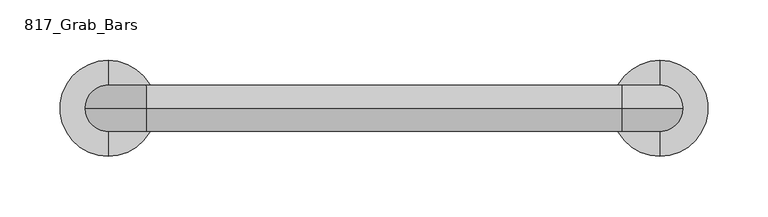
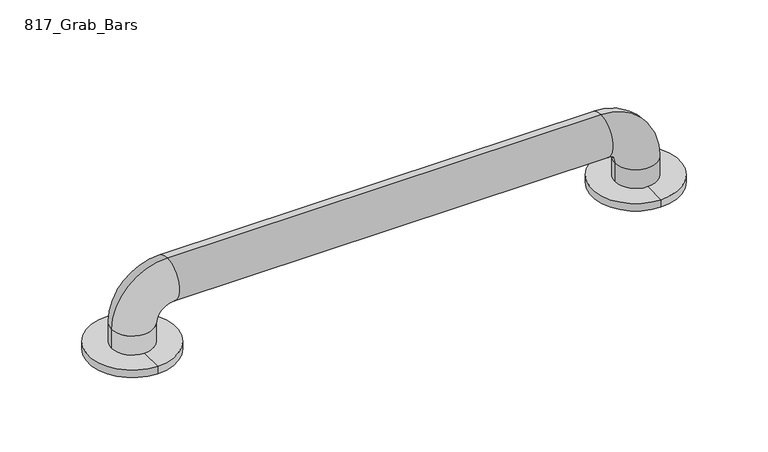
"""IFC4 building model written with IfcOpenShell, lengths in millimetres: proxy geometry, 817_Grab_Bars : 8170-001180."""

from ifc_helpers import new_model, si_unit, point, frame, origin, place, context, project, spatial, circle_curve, ellipse_curve, trimmed, source, transform, mapped, element, save
from ifc_brep_helpers import plane_surface, cylinder_surface, revolved_surface, advanced_brep


def proxy_817_grab_bars_5335159d(model_context):
    return source(origin(), model_context, "Body", "AdvancedBrep", [
        advanced_brep(
        [(-134.9375, -496.8875, 7.14375), (-134.9375, -576.2625, 7.14375), (-134.9375, -555.625, 7.14375), (-153.9875, -536.575, 7.14375), (-134.9375, -517.525, 7.14375), (-115.8875, -536.575, 7.14375), (-134.9375, -576.2625, 0.0), (-134.9375, -496.8875, 0.0), (-134.9375, -517.525, 0.0), (-134.9375, -536.575, 0.0), (-134.9375, -555.625, 0.0), (322.2625, -496.8875, 7.14375), (322.2625, -576.2625, 7.14375), (322.2625, -555.625, 7.14375), (303.2125, -536.575, 7.14375), (322.2625, -517.525, 7.14375), (341.3125, -536.575, 7.14375), (322.2625, -576.2625, 0.0), (322.2625, -496.8875, 0.0), (322.2625, -517.525, 0.0), (322.2625, -536.575, 0.0), (322.2625, -555.625, 0.0), (-153.9875, -536.575, 25.4), (-115.8875, -536.575, 25.4), (-103.1875, -536.575, 76.2), (-103.1875, -536.575, 38.1), (290.5125, -536.575, 76.2), (290.5125, -536.575, 38.1), (341.3125, -536.575, 25.4), (303.2125, -536.575, 25.4)],
        [
            (0, 1, circle_curve(frame((-134.9375, -536.575, 7.14375), z_axis=(0.0, 0.0, 1.0), x_axis=(0.0, 1.0, 0.0)), 39.6875)),
            (1, 2),
            (2, 3, circle_curve(frame((-134.9375, -536.575, 7.14375), z_axis=(0.0, 0.0, -1.0), x_axis=(1.0, 0.0, 0.0)), 19.05)),
            (3, 4, circle_curve(frame((-134.9375, -536.575, 7.14375), z_axis=(0.0, 0.0, -1.0), x_axis=(1.0, 0.0, 0.0)), 19.05)),
            (4, 0),
            (1, 0, circle_curve(frame((-134.9375, -536.575, 7.14375), z_axis=(0.0, 0.0, 1.0), x_axis=(0.0, 1.0, 0.0)), 39.6875)),
            (4, 5, circle_curve(frame((-134.9375, -536.575, 7.14375), z_axis=(0.0, 0.0, -1.0), x_axis=(1.0, 0.0, 0.0)), 19.05)),
            (5, 2, circle_curve(frame((-134.9375, -536.575, 7.14375), z_axis=(0.0, 0.0, -1.0), x_axis=(1.0, 0.0, 0.0)), 19.05)),
            (6, 7, circle_curve(frame((-134.9375, -536.575, 0.0), z_axis=(0.0, 0.0, -1.0), x_axis=(0.0, 1.0, 0.0)), 39.6875)),
            (7, 8),
            (8, 9),
            (9, 10),
            (10, 6),
            (7, 6, circle_curve(frame((-134.9375, -536.575, 0.0), z_axis=(0.0, 0.0, -1.0), x_axis=(0.0, 1.0, 0.0)), 39.6875)),
            (0, 7),
            (6, 1),
            (11, 12, circle_curve(frame((322.2625, -536.575, 7.14375), z_axis=(0.0, 0.0, 1.0), x_axis=(0.0, 1.0, 0.0)), 39.6875)),
            (12, 13),
            (13, 14, circle_curve(frame((322.2625, -536.575, 7.14375), z_axis=(0.0, 0.0, -1.0), x_axis=(-1.0, 0.0, 0.0)), 19.05)),
            (14, 15, circle_curve(frame((322.2625, -536.575, 7.14375), z_axis=(0.0, 0.0, -1.0), x_axis=(-1.0, 0.0, 0.0)), 19.05)),
            (15, 11),
            (12, 11, circle_curve(frame((322.2625, -536.575, 7.14375), z_axis=(0.0, 0.0, 1.0), x_axis=(0.0, 1.0, 0.0)), 39.6875)),
            (15, 16, circle_curve(frame((322.2625, -536.575, 7.14375), z_axis=(0.0, 0.0, -1.0), x_axis=(-1.0, 0.0, 0.0)), 19.05)),
            (16, 13, circle_curve(frame((322.2625, -536.575, 7.14375), z_axis=(0.0, 0.0, -1.0), x_axis=(-1.0, 0.0, 0.0)), 19.05)),
            (17, 18, circle_curve(frame((322.2625, -536.575, 0.0), z_axis=(0.0, 0.0, -1.0), x_axis=(0.0, 1.0, 0.0)), 39.6875)),
            (18, 19),
            (19, 20),
            (20, 21),
            (21, 17),
            (18, 17, circle_curve(frame((322.2625, -536.575, 0.0), z_axis=(0.0, 0.0, -1.0), x_axis=(0.0, 1.0, 0.0)), 39.6875)),
            (11, 18),
            (17, 12),
            (22, 23, circle_curve(frame((-134.9375, -536.575, 25.4), z_axis=(0.0, 0.0, -1.0), x_axis=(1.0, 0.0, 0.0)), 19.05)),
            (23, 5),
            (3, 22),
            (23, 22, circle_curve(frame((-134.9375, -536.575, 25.4), z_axis=(0.0, 0.0, -1.0), x_axis=(1.0, 0.0, 0.0)), 19.05)),
            (22, 24, circle_curve(frame((-103.1875, -536.575, 25.4), z_axis=(0.0, 1.0, 0.0), x_axis=(-1.0, 0.0, 0.0)), 50.8)),
            (24, 25, circle_curve(frame((-103.1875, -536.575, 57.15), z_axis=(-1.0, 0.0, 0.0), x_axis=(0.0, 0.0, -1.0)), 19.05)),
            (25, 23, circle_curve(frame((-103.1875, -536.575, 25.4), z_axis=(0.0, -1.0, 0.0), x_axis=(-1.0, 0.0, 0.0)), 12.7)),
            (25, 24, circle_curve(frame((-103.1875, -536.575, 57.15), z_axis=(-1.0, 0.0, 0.0), x_axis=(0.0, 0.0, -1.0)), 19.05)),
            (24, 26),
            (26, 27, circle_curve(frame((290.5125, -536.575, 57.15), z_axis=(-1.0, 0.0, 0.0), x_axis=(0.0, 0.0, -1.0)), 19.05)),
            (27, 25),
            (27, 26, circle_curve(frame((290.5125, -536.575, 57.15), z_axis=(-1.0, 0.0, 0.0), x_axis=(0.0, 0.0, -1.0)), 19.05)),
            (26, 28, circle_curve(frame((290.5125, -536.575, 25.4), z_axis=(0.0, 1.0, 0.0), x_axis=(0.0, 0.0, 1.0)), 50.8)),
            (28, 29, circle_curve(frame((322.2625, -536.575, 25.4), z_axis=(0.0, 0.0, 1.0), x_axis=(-1.0, 0.0, 0.0)), 19.05)),
            (29, 27, circle_curve(frame((290.5125, -536.575, 25.4), z_axis=(0.0, -1.0, 0.0), x_axis=(0.0, 0.0, 1.0)), 12.7)),
            (29, 28, circle_curve(frame((322.2625, -536.575, 25.4), z_axis=(0.0, 0.0, 1.0), x_axis=(-1.0, 0.0, 0.0)), 19.05)),
            (28, 16),
            (14, 29),
        ],
        [
            plane_surface(frame((-134.9375, -536.575, 7.14375), z_axis=(0.0, 0.0, 1.0), x_axis=(0.0, 1.0, 0.0))),
            plane_surface(frame((-134.9375, -536.575, 0.0), z_axis=(0.0, 0.0, -1.0), x_axis=(0.0, 1.0, 0.0))),
            cylinder_surface(frame((-134.9375, -536.575, 7.14375), z_axis=(0.0, 0.0, 1.0), x_axis=(0.0, 1.0, 0.0)), 39.6875),
            plane_surface(frame((322.2625, -536.575, 7.14375), z_axis=(0.0, 0.0, 1.0), x_axis=(0.0, 1.0, 0.0))),
            plane_surface(frame((322.2625, -536.575, 0.0), z_axis=(0.0, 0.0, -1.0), x_axis=(0.0, 1.0, 0.0))),
            cylinder_surface(frame((322.2625, -536.575, 31.75), z_axis=(0.0, 0.0, 1.0), x_axis=(0.0, 1.0, 0.0)), 39.6875),
            cylinder_surface(frame((-134.9375, -536.575, 0.0), z_axis=(0.0, 0.0, -1.0), x_axis=(1.0, 0.0, 0.0)), 19.05),
            revolved_surface(trimmed(ellipse_curve(frame((-134.9375, -536.575, 25.4), z_axis=(0.0, 0.0, -1.0), x_axis=(1.0, 0.0, 0.0)), 19.05, 19.05), [point((-153.9875, -536.575, 25.4))], [point((-115.8875, -536.575, 25.4))], True, "CARTESIAN"), (-103.1875, -536.575, 25.4), (0.0, 1.0, 0.0)),
            revolved_surface(trimmed(ellipse_curve(frame((-134.9375, -536.575, 25.4), z_axis=(0.0, 0.0, -1.0), x_axis=(1.0, 0.0, 0.0)), 19.05, 19.05), [point((-115.8875, -536.575, 25.4))], [point((-153.9875, -536.575, 25.4))], True, "CARTESIAN"), (-103.1875, -536.575, 25.4), (0.0, 1.0, 0.0)),
            cylinder_surface(frame((-103.1875, -536.575, 57.15), z_axis=(-1.0, 0.0, 0.0), x_axis=(0.0, 0.0, -1.0)), 19.05),
            revolved_surface(trimmed(ellipse_curve(frame((290.5125, -536.575, 57.15), z_axis=(-1.0, 0.0, 0.0), x_axis=(0.0, 0.0, -1.0)), 19.05, 19.05), [point((290.5125, -536.575, 76.2))], [point((290.5125, -536.575, 38.1))], True, "CARTESIAN"), (290.5125, -536.575, 25.4), (0.0, 1.0, 0.0)),
            revolved_surface(trimmed(ellipse_curve(frame((290.5125, -536.575, 57.15), z_axis=(-1.0, 0.0, 0.0), x_axis=(0.0, 0.0, -1.0)), 19.05, 19.05), [point((290.5125, -536.575, 38.1))], [point((290.5125, -536.575, 76.2))], True, "CARTESIAN"), (290.5125, -536.575, 25.4), (0.0, 1.0, 0.0)),
            cylinder_surface(frame((322.2625, -536.575, 25.4), z_axis=(0.0, 0.0, 1.0), x_axis=(-1.0, 0.0, 0.0)), 19.05),
        ],
        [
            (0, [[1, 2, 3, 4, 5]]),
            (0, [[6, -5, 7, 8, -2]]),
            (1, [[9, 10, 11, 12, 13]]),
            (1, [[14, -13, -12, -11, -10]]),
            (2, [[-1, 15, -9, 16]]),
            (2, [[-6, -16, -14, -15]]),
            (3, [[17, 18, 19, 20, 21]]),
            (3, [[22, -21, 23, 24, -18]]),
            (4, [[25, 26, 27, 28, 29]]),
            (4, [[30, -29, -28, -27, -26]]),
            (5, [[-17, 31, -25, 32]]),
            (5, [[-22, -32, -30, -31]]),
            (6, [[33, 34, -7, -4, 35]]),
            (6, [[36, -35, -3, -8, -34]]),
            (7, [[-33, 37, 38, 39]]),
            (8, [[-36, -39, 40, -37]]),
            (9, [[-38, 41, 42, 43]]),
            (9, [[-40, -43, 44, -41]]),
            (10, [[-42, 45, 46, 47]]),
            (11, [[-44, -47, 48, -45]]),
            (12, [[-46, 49, -23, -20, 50]]),
            (12, [[-48, -50, -19, -24, -49]]),
        ],
    ),
    ])


if __name__ == "__main__":
    model = new_model("IFC4")
    model_context = context("Model", 3, world=origin())
    ifc_project = project(units=[si_unit("LENGTHUNIT", "METRE", prefix="MILLI")], contexts=[model_context])
    site = spatial("IfcSite", under=ifc_project)
    building = spatial("IfcBuilding", under=site)
    placement = place(None, origin())
    proxy_817_grab_bars_shape = proxy_817_grab_bars_5335159d(model_context)
    element("IfcBuildingElementProxy", 1, Name="817_Grab_Bars : 8170-001180", ObjectType="817_Grab_Bars : 8170-001180", at=placement, inside=building, context=model_context, shape_type="MappedRepresentation", body=[
        mapped(proxy_817_grab_bars_shape, transform((0.0, 0.0, 0.0), x_axis=(1.0, 0.0, 0.0), y_axis=(0.0, 1.0, 0.0), z_axis=(0.0, 0.0, 1.0))),
    ])
    save(model, "model.ifc")

# Revit data of these elements
# Type "817_Grab_Bars : 8170-001180"
#   Keynote = "M10281313.01"
#   Warranty Information = "Complete unit, one (1) year"
#   Version = "1.0"
#   Technical Data = "http://www.bradleycorp.com/products/techdata/8815.pdf"
#   URL = "www.bradleycorp.com"
#   Type Comments = "All grab bar configurations are specified using centerline to centerline dimensions."
#   OmniClass Title = ""
#   Modeling Code = ""
#   Model = "8170-001180"
#   Material Note = "FLANGES - 11 GA., TUBING - 18 GA."
#   MasterFormat Section Title = ""
#   Manufacturer = "Bradley Corporation"
#   LEED Credit = ""
#   Instructions [instance default] = "This is a face mounted fixture."
#   Industry Standards = "ANSI Standard A117.1, ADA, ABA, ADAAG, UFAS"
#   Fire Rating = "None"
#   Description = "Grab Bars"
#   Copyright = "This Model Data is Property of Bradley Corporation"
#   Complies to NAFTA = "Yes"
#   Complies To Buy American Act = "Yes"
#   Assembly Code = "C1030200"
#   ADA Compliant = "Yes"
#   Radius = 0' - 0 3/4"
#   Percentage of Recycled Content = 48.77
#   Overall Length = 1' - 9 1/8"
#   OmniClass Number = 0
#   MasterFormat Section Number = 0
#   Length = 1' - 6"
#   Diameter = 0' - 1 1/2"
#   Default Elevation = 2' - 9"
#   Material and Finish = Bradley Corp Stainless Steel - Satin
# Element 1 (IfcBuildingElementProxy, "817_Grab_Bars : 8170-001180")
#   Materials on its faces: "Bradley Corp Stainless Steel - Satin"
# Materials
#   "Bradley Corp Stainless Steel - Satin": class "Metal", colour RGB 189 187 185, transparency 0, Manufacturer = "Bradley Corporation", URL = "www.bradleycorp.com", Description = "Stainless Steel - Satin Finish", Cost = 0
